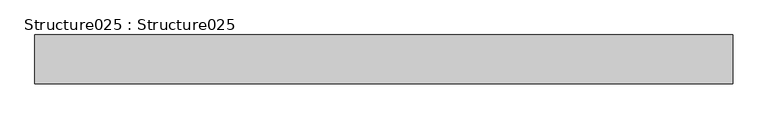
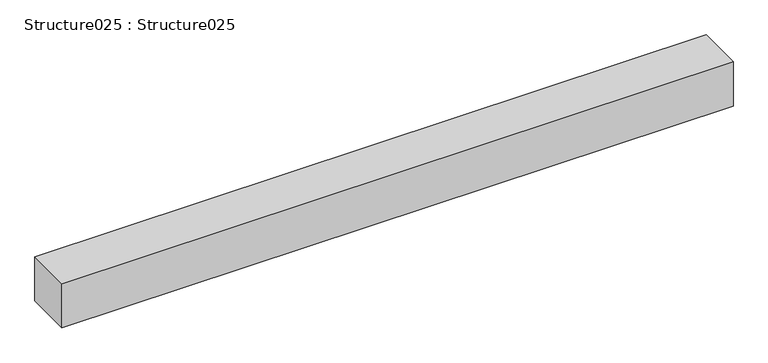
"""IFC4 building model written with IfcOpenShell, lengths in millimetres: proxy geometry, Structure025 : Structure025."""

from ifc_helpers import new_model, si_unit, frame, origin, place, context, project, spatial, polyline, outline, extrude, source, transform, mapped, element, save


def structure025_structure025_faa73e0b(model_context):
    return source(origin(), model_context, "Body", "SweptSolid", [
        extrude(outline(polyline([(14383.0178845, -4250.2279008), (14383.0178845, -4389.9279008), (12383.0178845, -4389.9279008), (12383.0178845, -4250.2279008), (14383.0178845, -4250.2279008)])), frame((0.0, 0.0, 42601.896), z_axis=(0.0, 0.0, 1.0), x_axis=(1.0, 0.0, 0.0)), (0.0, 0.0, 1.0), 139.7),
    ])


if __name__ == "__main__":
    model = new_model("IFC4")
    model_context = context("Model", 3, world=origin())
    ifc_project = project(units=[si_unit("LENGTHUNIT", "METRE", prefix="MILLI")], contexts=[model_context])
    site = spatial("IfcSite", under=ifc_project)
    building = spatial("IfcBuilding", under=site)
    placement = place(None, origin())
    structure025_structure025_shape = structure025_structure025_faa73e0b(model_context)
    element("IfcBuildingElementProxy", 1, Name="Structure025 : Structure025", ObjectType="Structure025 : Structure025", at=placement, inside=building, context=model_context, shape_type="MappedRepresentation", body=[
        mapped(structure025_structure025_shape, transform((0.0, 0.0, 0.0), x_axis=(1.0, 0.0, 0.0), y_axis=(0.0, 1.0, 0.0), z_axis=(0.0, 0.0, 1.0))),
    ])
    save(model, "model.ifc")

# Revit data of these elements
# Type "Structure025 : Structure025"
#   NameOverride = "Structure025"
# Element 1 (IfcBuildingElementProxy, "Structure025 : Structure025")
#   Materials on its faces: "STRUCTURAL MEMBER (SEE STRUCTURAL DWGS)"
# Materials
#   "STRUCTURAL MEMBER (SEE STRUCTURAL DWGS)": class "Unassigned", colour RGB 176 134 95, transparency 0, Cost = 0
